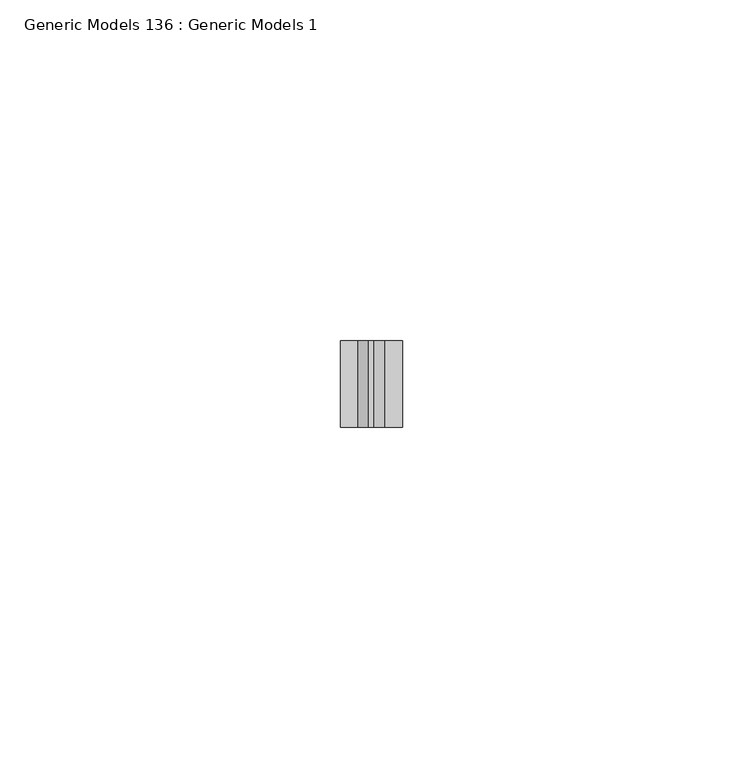
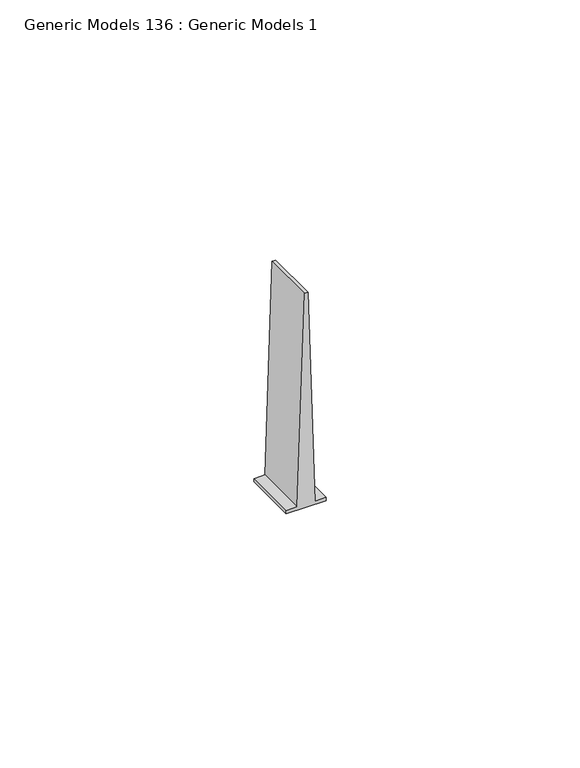
"""IFC4 building model written with IfcOpenShell, lengths in millimetres: proxy geometry, Generic Models 136 : Generic Models 1."""

from ifc_helpers import new_model, si_unit, frame, origin, place, context, project, spatial, polyline, outline, extrude, source, transform, mapped, element, save


def generic_models_136_generic_models_1_5c2c0c80(model_context):
    return source(origin(), model_context, "Body", "SweptSolid", [
        extrude(outline(polyline([(304.6453624, 49751.7340639), (304.6453624, 49760.8272639), (305.4391124, 49760.8272639), (305.4391124, 49758.2774003), (356.2391124, 49756.6800112), (356.2391124, 49755.8813166), (305.4391124, 49754.2839275), (305.4391124, 49751.7340639), (304.6453624, 49751.7340639)])), frame((0.0, 565.15, 0.0), z_axis=(0.0, 1.0, 0.0), x_axis=(0.0, 0.0, 1.0)), (0.0, 0.0, 1.0), 12.7),
    ])


if __name__ == "__main__":
    model = new_model("IFC4")
    model_context = context("Model", 3, world=origin())
    ifc_project = project(units=[si_unit("LENGTHUNIT", "METRE", prefix="MILLI")], contexts=[model_context])
    site = spatial("IfcSite", under=ifc_project)
    building = spatial("IfcBuilding", under=site)
    placement = place(None, origin())
    generic_models_136_generic_models_1_shape = generic_models_136_generic_models_1_5c2c0c80(model_context)
    element("IfcBuildingElementProxy", 1, Name="Generic Models 136 : Generic Models 1", ObjectType="Generic Models 136 : Generic Models 1", at=placement, inside=building, context=model_context, shape_type="MappedRepresentation", body=[
        mapped(generic_models_136_generic_models_1_shape, transform((0.0, 0.0, 0.0), x_axis=(1.0, 0.0, 0.0), y_axis=(0.0, 1.0, 0.0), z_axis=(0.0, 0.0, 1.0))),
    ])
    save(model, "model.ifc")

# Revit data of these elements
# Element 1 (IfcBuildingElementProxy, "Generic Models 136 : Generic Models 1")
#   Materials on its faces: "METAL RUNNER CHANNEL; FASTEN @ 24\" O.C."
# Materials
#   "METAL RUNNER CHANNEL; FASTEN @ 24\" O.C.": class "Unassigned", colour RGB 210 209 208, transparency 0, Keynote = "M05121300.02", Cost = 0
